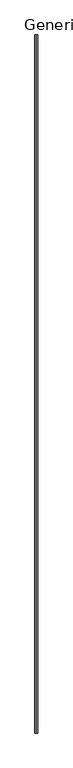
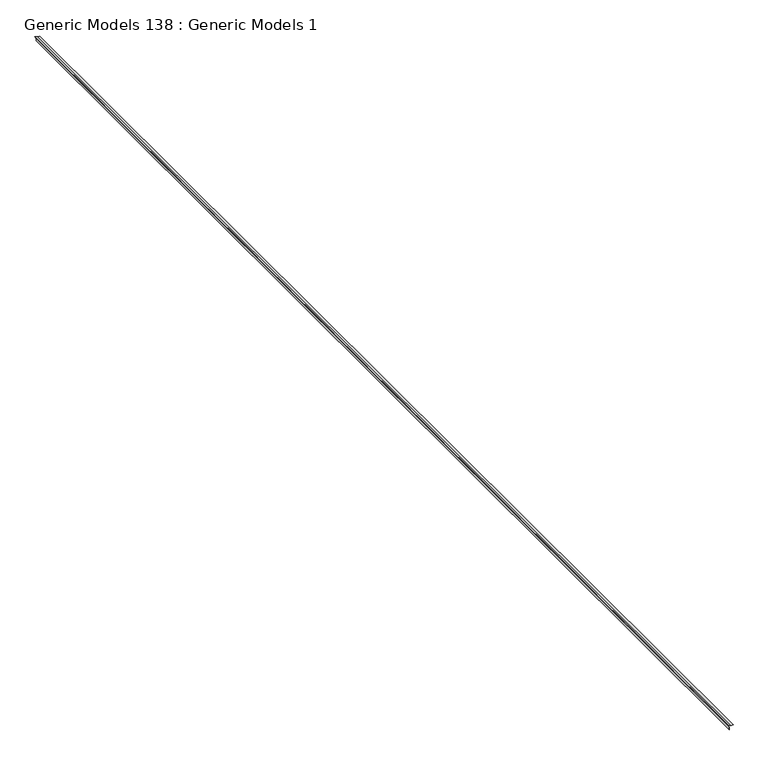
"""IFC4 building model written with IfcOpenShell, lengths in millimetres: proxy geometry, Generic Models 138 : Generic Models 1."""

from ifc_helpers import new_model, si_unit, point, frame, frame_2d, origin, place, context, project, spatial, polyline, circle_curve, trimmed, segment, composite_curve, outline, extrude, source, transform, mapped, element, save


def generic_models_138_generic_models_1_829eee8d(model_context):
    return source(origin(), model_context, "Body", "SweptSolid", [
        extrude(outline(composite_curve([segment(trimmed(circle_curve(frame_2d((127127.2167873, 7060.4457008)), 1.4342127), [point((127128.4926156, 7061.1008558))], [point((127126.5616323, 7059.1698725))], False, "CARTESIAN"), True, "CONTINUOUS"), segment(polyline([(127126.5616323, 7059.1698725), (127088.5361176, 7078.6964881), (127050.4361176, 7078.6964881), (127050.4361176, 7079.9664881), (127088.8431414, 7079.9664881), (127127.5962396, 7060.0662484), (127107.696, 7098.8193467), (127107.696, 7137.2263705), (127108.966, 7137.2263705), (127108.966, 7099.1263705), (127128.4926156, 7061.1008558)]), True, "CONTINUOUS")], self_intersect=False)), frame((0.0, -7068.1230338, 0.0), z_axis=(0.0, 1.0, 0.0), x_axis=(0.0, 0.0, 1.0)), (0.0, 0.0, 1.0), 19050.0),
    ])


if __name__ == "__main__":
    model = new_model("IFC4")
    model_context = context("Model", 3, world=origin())
    ifc_project = project(units=[si_unit("LENGTHUNIT", "METRE", prefix="MILLI")], contexts=[model_context])
    site = spatial("IfcSite", under=ifc_project)
    building = spatial("IfcBuilding", under=site)
    placement = place(None, origin())
    generic_models_138_generic_models_1_shape = generic_models_138_generic_models_1_829eee8d(model_context)
    element("IfcBuildingElementProxy", 1, Name="Generic Models 138 : Generic Models 1", ObjectType="Generic Models 138 : Generic Models 1", at=placement, inside=building, context=model_context, shape_type="MappedRepresentation", body=[
        mapped(generic_models_138_generic_models_1_shape, transform((0.0, 0.0, 0.0), x_axis=(1.0, 0.0, 0.0), y_axis=(0.0, 1.0, 0.0), z_axis=(0.0, 0.0, 1.0))),
    ])
    save(model, "model.ifc")

# Revit data of these elements
# Element 1 (IfcBuildingElementProxy, "Generic Models 138 : Generic Models 1")
#   Materials on its faces: "_CONTINUOUS 16 GA. COPPER CORNER BEAD"
# Materials
#   "_CONTINUOUS 16 GA. COPPER CORNER BEAD": class "Generic", colour RGB 253 192 103, transparency 0, Cost = 0
